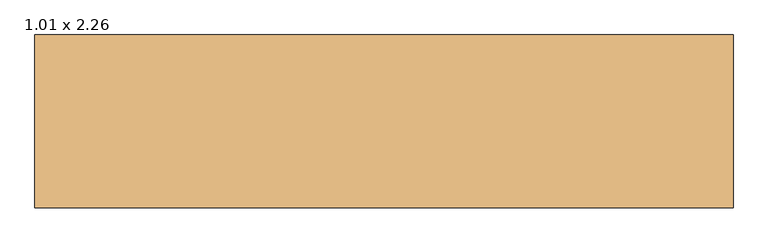
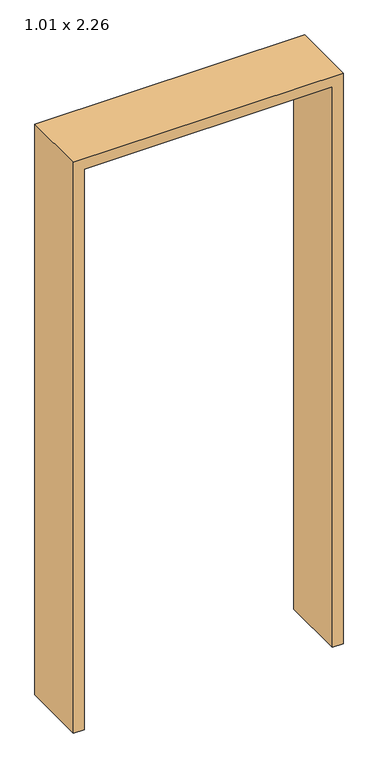
"""IFC4 building model written with IfcOpenShell, lengths in millimetres: door geometry, Durchfahrt - Blockzarge : 1.01 x 2.26."""

from ifc_helpers import new_model, si_unit, frame, origin, place, context, project, spatial, polyline, outline, extrude, source, transform, mapped, element, save


def door_1_01_x_2_26_f360ade5(model_context):
    return source(origin(), model_context, "Body", "SweptSolid", [
        extrude(outline(polyline([(2360.0, 505.0), (2360.0, -505.0), (100.0, -505.0), (100.0, -465.0), (2320.0, -465.0), (2320.0, 465.0), (100.0, 465.0), (100.0, 505.0), (2360.0, 505.0)])), frame((0.0, -110.5653859, 0.0), z_axis=(0.0, 1.0, 0.0), x_axis=(0.0, 0.0, 1.0)), (0.0, 0.0, 1.0), 250.0),
    ])


if __name__ == "__main__":
    model = new_model("IFC4")
    model_context = context("Model", 3, world=origin())
    ifc_project = project(units=[si_unit("LENGTHUNIT", "METRE", prefix="MILLI")], contexts=[model_context])
    site = spatial("IfcSite", under=ifc_project)
    building = spatial("IfcBuilding", under=site)
    placement = place(None, origin())
    door_1_01_x_2_26_shape = door_1_01_x_2_26_f360ade5(model_context)
    element("IfcDoor", 1, ObjectType="Durchfahrt - Blockzarge : 1.01 x 2.26", at=placement, inside=building, context=model_context, shape_type="MappedRepresentation", body=[
        mapped(door_1_01_x_2_26_shape, transform((0.0, 0.0, 0.0), x_axis=(1.0, 0.0, 0.0), y_axis=(0.0, 1.0, 0.0), z_axis=(0.0, 0.0, 1.0))),
    ])
    save(model, "model.ifc")

# Revit data of these elements
# Type "Durchfahrt - Blockzarge : 1.01 x 2.26"
#   Type Mark = "22"
#   Keynote = "16.03"
#   Rough Width = 1.010 m
#   Stärke Futter = 0.040 m
#   Rough Height [instance default] = 2.360 m
#   Height = 2.260 m
#   Fußbodenaufbau [instance default] = 0.100 m
#   Width = 1.010 m
#   Sichtbarkeit Sturzlinien [instance default] = yes
#   Rahmen/Pfosten = none
#   Function = (empty or 0)
#   Wall Closure = (empty or 0)
# Element 1 (IfcDoor, "Durchfahrt - Blockzarge : 1.01 x 2.26")
#   Materials on its faces: "Holz - Birke"
# Materials
#   "Holz - Birke": class "Holz", colour RGB 213 164 103, transparency 0, Cost = 0
